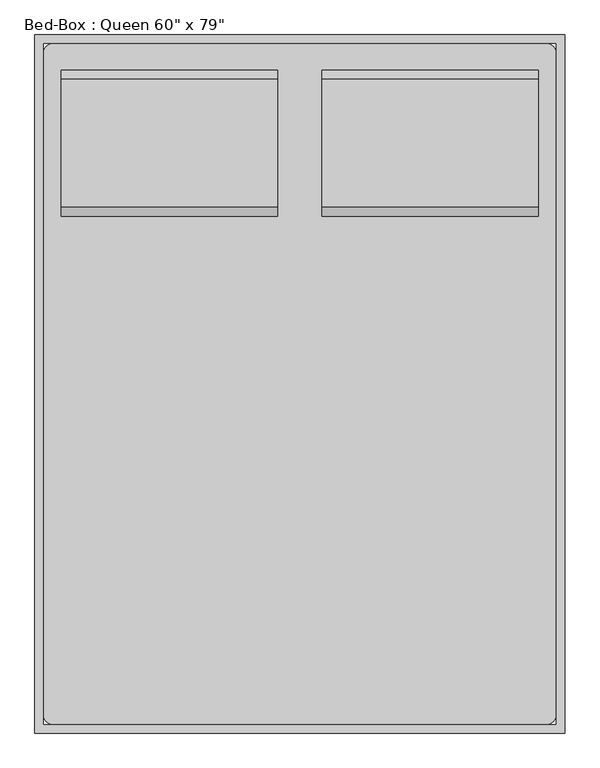
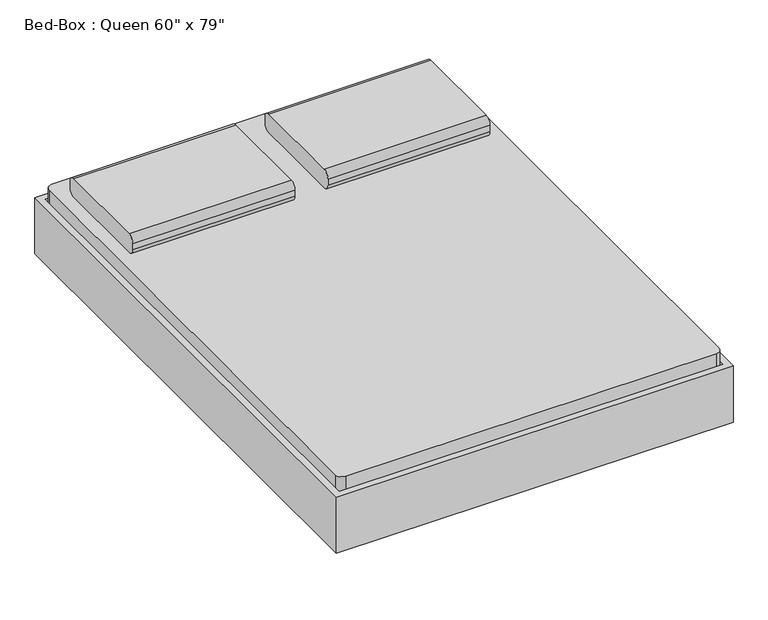
"""IFC4 building model written with IfcOpenShell, lengths in millimetres: furniture geometry."""

from ifc_helpers import new_model, si_unit, point, frame, frame_2d, origin, place, context, project, spatial, polyline, circle_curve, trimmed, segment, composite_curve, outline, extrude, source, transform, mapped, element, save
from ifc_brep_helpers import plane_surface, cylinder_surface, revolved_surface, advanced_brep


def furniture_0fd752b5(model_context):
    return source(origin(), model_context, "Body", "SolidModel", [
        extrude(outline(composite_curve([segment(polyline([(641.8704918, 406.4), (273.5704918, 406.4)]), True, "CONTINUOUS"), segment(trimmed(circle_curve(frame_2d((273.5704918, 431.8)), 25.4), [point((273.5704918, 406.4))], [point((248.1704918, 431.8))], False, "CARTESIAN"), True, "CONTINUOUS"), segment(polyline([(248.1704918, 431.8), (248.1704918, 457.2)]), True, "CONTINUOUS"), segment(trimmed(circle_curve(frame_2d((273.5704918, 457.2)), 25.4), [point((248.1704918, 457.2))], [point((273.5704918, 482.6))], False, "CARTESIAN"), True, "CONTINUOUS"), segment(polyline([(273.5704918, 482.6), (641.8704918, 482.6)]), True, "CONTINUOUS"), segment(trimmed(circle_curve(frame_2d((641.8704918, 457.2)), 25.4), [point((641.8704918, 482.6))], [point((667.2704918, 457.2))], False, "CARTESIAN"), True, "CONTINUOUS"), segment(polyline([(667.2704918, 457.2), (667.2704918, 431.8)]), True, "CONTINUOUS"), segment(trimmed(circle_curve(frame_2d((641.8704918, 431.8)), 25.4), [point((667.2704918, 431.8))], [point((641.8704918, 406.4))], False, "CARTESIAN"), True, "CONTINUOUS")], self_intersect=False)), frame((402.652459, 0.0, 0.0), z_axis=(1.0, 0.0, 0.0), x_axis=(0.0, 1.0, 0.0)), (0.0, 0.0, 1.0), 622.3),
        extrude(outline(composite_curve([segment(polyline([(641.8704918, 406.4), (273.5704918, 406.4)]), True, "CONTINUOUS"), segment(trimmed(circle_curve(frame_2d((273.5704918, 431.8)), 25.4), [point((273.5704918, 406.4))], [point((248.1704918, 431.8))], False, "CARTESIAN"), True, "CONTINUOUS"), segment(polyline([(248.1704918, 431.8), (248.1704918, 457.2)]), True, "CONTINUOUS"), segment(trimmed(circle_curve(frame_2d((273.5704918, 457.2)), 25.4), [point((248.1704918, 457.2))], [point((273.5704918, 482.6))], False, "CARTESIAN"), True, "CONTINUOUS"), segment(polyline([(273.5704918, 482.6), (641.8704918, 482.6)]), True, "CONTINUOUS"), segment(trimmed(circle_curve(frame_2d((641.8704918, 457.2)), 25.4), [point((641.8704918, 482.6))], [point((667.2704918, 457.2))], False, "CARTESIAN"), True, "CONTINUOUS"), segment(polyline([(667.2704918, 457.2), (667.2704918, 431.8)]), True, "CONTINUOUS"), segment(trimmed(circle_curve(frame_2d((641.8704918, 431.8)), 25.4), [point((667.2704918, 431.8))], [point((641.8704918, 406.4))], False, "CARTESIAN"), True, "CONTINUOUS")], self_intersect=False)), frame((-346.647541, 0.0, 0.0), z_axis=(1.0, 0.0, 0.0), x_axis=(0.0, 1.0, 0.0)), (0.0, 0.0, 1.0), 622.3),
        advanced_brep(
        [(-397.1231784, 514.8704918, 177.8), (-397.1231784, 438.6704918, 177.8), (-397.1231784, 438.6704918, 196.85), (-397.1231784, 514.8704918, 196.85), (-346.3231784, 514.8704918, 177.8), (-346.3231784, 438.6704918, 177.8), (-334.1869899, 438.6704918, 196.85), (-334.1869899, 514.8704918, 196.85), (-270.2523099, 514.8704918, 14.6654962), (-270.2523099, 438.6704918, 14.6654962), (-252.9871466, 438.6704918, 22.716374), (-252.9871466, 514.8704918, 22.716374), (-247.2320921, 438.6704918, 0.0), (-247.2320921, 514.8704918, 0.0), (-247.2320921, 438.6704918, 19.05), (-247.2320921, 514.8704918, 19.05), (-168.6195862, 514.8704918, 0.0), (-168.6195862, 438.6704918, 0.0), (-168.6195862, 438.6704918, 19.05), (-168.6195862, 514.8704918, 19.05), (-155.9195862, 438.6704918, 3.4029547), (-155.9195862, 514.8704918, 3.4029547), (-165.4445862, 438.6704918, 19.9007387), (-165.4445862, 514.8704918, 19.9007387), (-95.822541, 514.8704918, 38.1), (-95.822541, 438.6704918, 38.1), (-100.9269731, 438.6704918, 57.15), (-100.9269731, 514.8704918, 57.15), (774.4518216, 514.8704918, 38.1), (774.4518216, 438.6704918, 38.1), (779.5562537, 438.6704918, 57.15), (779.5562537, 514.8704918, 57.15), (834.5488669, 514.8704918, 3.4029547), (834.5488669, 438.6704918, 3.4029547), (844.0738669, 438.6704918, 19.9007387), (844.0738669, 514.8704918, 19.9007387), (847.2488669, 438.6704918, 0.0), (847.2488669, 514.8704918, 0.0), (847.2488669, 438.6704918, 19.05), (847.2488669, 514.8704918, 19.05), (925.8613728, 514.8704918, 0.0), (925.8613728, 438.6704918, 0.0), (925.8613728, 438.6704918, 19.05), (925.8613728, 514.8704918, 19.05), (948.8815906, 438.6704918, 14.6654962), (948.8815906, 514.8704918, 14.6654962), (931.6164272, 438.6704918, 22.716374), (931.6164272, 514.8704918, 22.716374), (1024.952459, 514.8704918, 177.8), (1024.952459, 438.6704918, 177.8), (1012.8162705, 438.6704918, 196.85), (1012.8162705, 514.8704918, 196.85), (1075.752459, 514.8704918, 177.8), (1075.752459, 514.8704918, 196.85), (1075.752459, 438.6704918, 196.85), (1075.752459, 438.6704918, 177.8)],
        [
            (0, 1),
            (1, 2),
            (2, 3),
            (3, 0),
            (0, 4),
            (4, 5),
            (5, 1),
            (5, 6),
            (6, 2),
            (6, 7),
            (7, 3),
            (7, 4),
            (4, 8),
            (8, 9),
            (9, 5),
            (9, 10),
            (10, 6),
            (10, 11),
            (11, 7),
            (11, 8),
            (12, 9, circle_curve(frame((-247.2320921, 438.6704918, 25.4), z_axis=(0.0, 1.0, 0.0), x_axis=(-0.9063077870366486, 0.0, -0.42261826174070233)), 25.4)),
            (8, 13, circle_curve(frame((-247.2320921, 514.8704918, 25.4), z_axis=(0.0, -1.0, 0.0), x_axis=(-0.9063077870366486, 0.0, -0.42261826174070233)), 25.4)),
            (13, 12),
            (14, 10, circle_curve(frame((-247.2320921, 438.6704918, 25.4), z_axis=(0.0, 1.0, 0.0), x_axis=(-0.9063077870366486, 0.0, -0.42261826174070233)), 6.35)),
            (12, 14),
            (15, 11, circle_curve(frame((-247.2320921, 514.8704918, 25.4), z_axis=(0.0, 1.0, 0.0), x_axis=(-0.9063077870366486, 0.0, -0.42261826174070233)), 6.35)),
            (14, 15),
            (15, 13),
            (13, 16),
            (16, 17),
            (17, 12),
            (17, 18),
            (18, 14),
            (18, 19),
            (19, 15),
            (19, 16),
            (20, 17, circle_curve(frame((-168.6195862, 438.6704918, 25.4), z_axis=(0.0, 1.0, 0.0), x_axis=(0.0, 0.0, -1.0)), 25.4)),
            (16, 21, circle_curve(frame((-168.6195862, 514.8704918, 25.4), z_axis=(0.0, -1.0, 0.0), x_axis=(0.0, 0.0, -1.0)), 25.4)),
            (21, 20),
            (22, 18, circle_curve(frame((-168.6195862, 438.6704918, 25.4), z_axis=(0.0, 1.0, 0.0), x_axis=(0.0, 0.0, -1.0)), 6.35)),
            (20, 22),
            (23, 19, circle_curve(frame((-168.6195862, 514.8704918, 25.4), z_axis=(0.0, 1.0, 0.0), x_axis=(0.0, 0.0, -1.0)), 6.35)),
            (22, 23),
            (23, 21),
            (21, 24),
            (24, 25),
            (25, 20),
            (25, 26),
            (26, 22),
            (26, 27),
            (27, 23),
            (27, 24),
            (24, 28),
            (28, 29),
            (29, 25),
            (29, 30),
            (30, 26),
            (30, 31),
            (31, 27),
            (31, 28),
            (28, 32),
            (32, 33),
            (33, 29),
            (33, 34),
            (34, 30),
            (34, 35),
            (35, 31),
            (35, 32),
            (36, 33, circle_curve(frame((847.2488669, 438.6704918, 25.4), z_axis=(0.0, 1.0, 0.0), x_axis=(-0.5000000000000463, 0.0, -0.8660254037844118)), 25.4)),
            (32, 37, circle_curve(frame((847.2488669, 514.8704918, 25.4), z_axis=(0.0, -1.0, 0.0), x_axis=(-0.5000000000000463, 0.0, -0.8660254037844118)), 25.4)),
            (37, 36),
            (38, 34, circle_curve(frame((847.2488669, 438.6704918, 25.4), z_axis=(0.0, 1.0, 0.0), x_axis=(-0.5000000000000463, 0.0, -0.8660254037844118)), 6.35)),
            (36, 38),
            (39, 35, circle_curve(frame((847.2488669, 514.8704918, 25.4), z_axis=(0.0, 1.0, 0.0), x_axis=(-0.5000000000000463, 0.0, -0.8660254037844118)), 6.35)),
            (38, 39),
            (39, 37),
            (37, 40),
            (40, 41),
            (41, 36),
            (41, 42),
            (42, 38),
            (42, 43),
            (43, 39),
            (43, 40),
            (44, 41, circle_curve(frame((925.8613728, 438.6704918, 25.4), z_axis=(0.0, 1.0, 0.0), x_axis=(0.0, 0.0, -1.0)), 25.4)),
            (40, 45, circle_curve(frame((925.8613728, 514.8704918, 25.4), z_axis=(0.0, -1.0, 0.0), x_axis=(0.0, 0.0, -1.0)), 25.4)),
            (45, 44),
            (46, 42, circle_curve(frame((925.8613728, 438.6704918, 25.4), z_axis=(0.0, 1.0, 0.0), x_axis=(0.0, 0.0, -1.0)), 6.35)),
            (44, 46),
            (47, 43, circle_curve(frame((925.8613728, 514.8704918, 25.4), z_axis=(0.0, 1.0, 0.0), x_axis=(0.0, 0.0, -1.0)), 6.35)),
            (46, 47),
            (47, 45),
            (45, 48),
            (48, 49),
            (49, 44),
            (49, 50),
            (50, 46),
            (50, 51),
            (51, 47),
            (51, 48),
            (52, 53),
            (53, 54),
            (54, 55),
            (55, 52),
            (48, 52),
            (55, 49),
            (54, 50),
            (53, 51),
        ],
        [
            plane_surface(frame((-397.1231784, 768.8704918, -152.9490627), z_axis=(-1.0, 0.0, 0.0), x_axis=(0.0, 1.0, 0.0))),
            plane_surface(frame((-397.1231784, 514.8704918, 177.8), z_axis=(0.0, 0.0, -1.0), x_axis=(1.0, 0.0, 0.0))),
            plane_surface(frame((-397.1231784, 438.6704918, 177.8), z_axis=(0.0, -1.0, 0.0), x_axis=(1.0, 0.0, 0.0))),
            plane_surface(frame((-397.1231784, 438.6704918, 196.85), z_axis=(0.0, 0.0, 1.0), x_axis=(1.0, 0.0, 0.0))),
            plane_surface(frame((-397.1231784, 514.8704918, 196.85), z_axis=(0.0, 1.0, 0.0), x_axis=(1.0, 0.0, 0.0))),
            plane_surface(frame((-346.3231784, 514.8704918, 177.8), z_axis=(-0.9063077870366485, 0.0, -0.4226182617407027), x_axis=(0.4226182617407027, 0.0, -0.9063077870366485))),
            plane_surface(frame((-346.3231784, 438.6704918, 177.8), z_axis=(0.0, -1.0, 0.0), x_axis=(0.4226182617407025, 0.0, -0.9063077870366486))),
            plane_surface(frame((-334.1869899, 438.6704918, 196.85), z_axis=(0.9063077870366484, 0.0, 0.4226182617407028), x_axis=(0.4226182617407028, 0.0, -0.9063077870366484))),
            plane_surface(frame((-334.1869899, 514.8704918, 196.85), z_axis=(0.0, 1.0, 0.0), x_axis=(0.42261826174070277, 0.0, -0.9063077870366485))),
            cylinder_surface(frame((-247.2320921, 768.8704918, 25.4), z_axis=(0.0, -1.0, 0.0), x_axis=(-0.9063077870366486, 0.0, -0.42261826174070233)), 25.4),
            plane_surface(frame((-247.2320921, 438.6704918, 25.4), z_axis=(0.0, -1.0, 0.0), x_axis=(-0.9063077870366486, 0.0, -0.42261826174070233))),
            revolved_surface(polyline([(-252.9871465476827, 438.6704918, 22.71637403794654), (-252.9871465476827, 514.8704918, 22.71637403794654)]), (-247.2320921, 768.8704918, 25.4), (0.0, -1.0, 0.0)),
            plane_surface(frame((-247.2320921, 514.8704918, 25.4), z_axis=(0.0, 1.0, 0.0), x_axis=(-0.9063077870366486, 0.0, -0.42261826174070233))),
            plane_surface(frame((-247.2320921, 514.8704918, 0.0), z_axis=(0.0, 0.0, -1.0), x_axis=(1.0, 0.0, 0.0))),
            plane_surface(frame((-247.2320921, 438.6704918, 0.0), z_axis=(0.0, -1.0, 0.0), x_axis=(1.0, 0.0, 0.0))),
            plane_surface(frame((-247.2320921, 438.6704918, 19.05), z_axis=(0.0, 0.0, 1.0), x_axis=(1.0, 0.0, 0.0))),
            plane_surface(frame((-247.2320921, 514.8704918, 19.05), z_axis=(0.0, 1.0, 0.0), x_axis=(1.0, 0.0, 0.0))),
            cylinder_surface(frame((-168.6195862, 768.8704918, 25.4), z_axis=(0.0, -1.0, 0.0), x_axis=(0.0, 0.0, -1.0)), 25.4),
            plane_surface(frame((-168.6195862, 438.6704918, 25.4), z_axis=(0.0, -1.0, 0.0), x_axis=(0.0, 0.0, -1.0))),
            revolved_surface(polyline([(-168.6195862, 438.6704918, 19.049999999999997), (-168.6195862, 514.8704918, 19.049999999999997)]), (-168.6195862, 768.8704918, 25.4), (0.0, -1.0, 0.0)),
            plane_surface(frame((-168.6195862, 514.8704918, 25.4), z_axis=(0.0, 1.0, 0.0), x_axis=(0.0, 0.0, -1.0))),
            plane_surface(frame((-155.9195862, 514.8704918, 3.4029547), z_axis=(0.49999999999988004, 0.0, -0.866025403784508), x_axis=(0.866025403784508, 0.0, 0.49999999999988004))),
            plane_surface(frame((-155.9195862, 438.6704918, 3.4029547), z_axis=(0.0, -1.0, 0.0), x_axis=(0.8660254037845078, 0.0, 0.49999999999988026))),
            plane_surface(frame((-165.4445862, 438.6704918, 19.9007387), z_axis=(-0.4999999999998799, 0.0, 0.866025403784508), x_axis=(0.866025403784508, 0.0, 0.4999999999998799))),
            plane_surface(frame((-165.4445862, 514.8704918, 19.9007387), z_axis=(0.0, 1.0, 0.0), x_axis=(0.8660254037845075, 0.0, 0.49999999999988076))),
            plane_surface(frame((-95.822541, 514.8704918, 38.1), z_axis=(0.0, 0.0, -1.0), x_axis=(1.0, 0.0, 0.0))),
            plane_surface(frame((-95.822541, 438.6704918, 38.1), z_axis=(0.0, -1.0, 0.0), x_axis=(1.0, 0.0, 0.0))),
            plane_surface(frame((-100.9269731, 438.6704918, 57.15), z_axis=(0.0, 0.0, 1.0), x_axis=(1.0, 0.0, 0.0))),
            plane_surface(frame((-100.9269731, 514.8704918, 57.15), z_axis=(0.0, 1.0, 0.0), x_axis=(1.0, 0.0, 0.0))),
            plane_surface(frame((774.4518216, 514.8704918, 38.1), z_axis=(-0.5000000000000455, 0.0, -0.8660254037844125), x_axis=(0.8660254037844125, 0.0, -0.5000000000000455))),
            plane_surface(frame((774.4518216, 438.6704918, 38.1), z_axis=(0.0, -1.0, 0.0), x_axis=(0.866025403784412, 0.0, -0.5000000000000463))),
            plane_surface(frame((779.5562537, 438.6704918, 57.15), z_axis=(0.5000000000000466, 0.0, 0.8660254037844117), x_axis=(0.8660254037844117, 0.0, -0.5000000000000466))),
            plane_surface(frame((779.5562537, 514.8704918, 57.15), z_axis=(0.0, 1.0, 0.0), x_axis=(0.8660254037844115, 0.0, -0.5000000000000471))),
            cylinder_surface(frame((847.2488669, 768.8704918, 25.4), z_axis=(0.0, -1.0, 0.0), x_axis=(-0.5000000000000463, 0.0, -0.8660254037844118)), 25.4),
            plane_surface(frame((847.2488669, 438.6704918, 25.4), z_axis=(0.0, -1.0000000000000002, 0.0), x_axis=(-0.5000000000000464, 0.0, -0.866025403784412))),
            revolved_surface(polyline([(844.0738668999998, 438.6704918, 19.90073868596898), (844.0738668999998, 514.8704918, 19.90073868596898)]), (847.2488669, 768.8704918, 25.4), (0.0, -1.0, 0.0)),
            plane_surface(frame((847.2488669, 514.8704918, 25.4), z_axis=(0.0, 1.0000000000000002, 0.0), x_axis=(-0.5000000000000464, 0.0, -0.866025403784412))),
            plane_surface(frame((847.2488669, 514.8704918, 0.0), z_axis=(0.0, 0.0, -1.0), x_axis=(1.0, 0.0, 0.0))),
            plane_surface(frame((847.2488669, 438.6704918, 0.0), z_axis=(0.0, -1.0, 0.0), x_axis=(1.0, 0.0, 0.0))),
            plane_surface(frame((847.2488669, 438.6704918, 19.05), z_axis=(0.0, 0.0, 1.0), x_axis=(1.0, 0.0, 0.0))),
            plane_surface(frame((847.2488669, 514.8704918, 19.05), z_axis=(0.0, 1.0, 0.0), x_axis=(1.0, 0.0, 0.0))),
            cylinder_surface(frame((925.8613728, 768.8704918, 25.4), z_axis=(0.0, -1.0, 0.0), x_axis=(0.0, 0.0, -1.0)), 25.4),
            plane_surface(frame((925.8613728, 438.6704918, 25.4), z_axis=(0.0, -1.0, 0.0), x_axis=(0.0, 0.0, -1.0))),
            revolved_surface(polyline([(925.8613728, 438.6704918, 19.049999999999997), (925.8613728, 514.8704918, 19.049999999999997)]), (925.8613728, 768.8704918, 25.4), (0.0, -1.0, 0.0)),
            plane_surface(frame((925.8613728, 514.8704918, 25.4), z_axis=(0.0, 1.0, 0.0), x_axis=(0.0, 0.0, -1.0))),
            plane_surface(frame((948.8815906, 514.8704918, 14.6654962), z_axis=(0.90630778703668, 0.0, -0.42261826174063527), x_axis=(0.42261826174063527, 0.0, 0.90630778703668))),
            plane_surface(frame((948.8815906, 438.6704918, 14.6654962), z_axis=(0.0, -1.0, 0.0), x_axis=(0.42261826174063566, 0.0, 0.9063077870366797))),
            plane_surface(frame((931.6164272, 438.6704918, 22.716374), z_axis=(-0.9063077870366801, 0.0, 0.4226182617406349), x_axis=(0.4226182617406349, 0.0, 0.9063077870366801))),
            plane_surface(frame((931.6164272, 514.8704918, 22.716374), z_axis=(0.0, 1.0, 0.0), x_axis=(0.4226182617406353, 0.0, 0.9063077870366799))),
            plane_surface(frame((1075.752459, 768.8704918, -152.9490627), z_axis=(1.0, 0.0, 0.0), x_axis=(0.0, 1.0, 0.0))),
            plane_surface(frame((1024.952459, 514.8704918, 177.8), z_axis=(0.0, 0.0, -1.0), x_axis=(1.0, 0.0, 0.0))),
            plane_surface(frame((1024.952459, 438.6704918, 177.8), z_axis=(0.0, -1.0, 0.0), x_axis=(1.0, 0.0, 0.0))),
            plane_surface(frame((1012.8162705, 438.6704918, 196.85), z_axis=(0.0, 0.0, 1.0), x_axis=(1.0, 0.0, 0.0))),
            plane_surface(frame((1012.8162705, 514.8704918, 196.85), z_axis=(0.0, 1.0, 0.0), x_axis=(1.0, 0.0, 0.0))),
        ],
        [
            (0, [[1, 2, 3, 4]]),
            (1, [[-1, 5, 6, 7]]),
            (2, [[-2, -7, 8, 9]]),
            (3, [[-3, -9, 10, 11]]),
            (4, [[-4, -11, 12, -5]]),
            (5, [[-6, 13, 14, 15]]),
            (6, [[-8, -15, 16, 17]]),
            (7, [[-10, -17, 18, 19]]),
            (8, [[-12, -19, 20, -13]]),
            (9, [[21, -14, 22, 23]]),
            (10, [[24, -16, -21, 25]]),
            (11, [[26, -18, -24, 27]]),
            (12, [[-22, -20, -26, 28]]),
            (13, [[-23, 29, 30, 31]]),
            (14, [[-25, -31, 32, 33]]),
            (15, [[-27, -33, 34, 35]]),
            (16, [[-28, -35, 36, -29]]),
            (17, [[37, -30, 38, 39]]),
            (18, [[40, -32, -37, 41]]),
            (19, [[42, -34, -40, 43]]),
            (20, [[-38, -36, -42, 44]]),
            (21, [[-39, 45, 46, 47]]),
            (22, [[-41, -47, 48, 49]]),
            (23, [[-43, -49, 50, 51]]),
            (24, [[-44, -51, 52, -45]]),
            (25, [[-46, 53, 54, 55]]),
            (26, [[-48, -55, 56, 57]]),
            (27, [[-50, -57, 58, 59]]),
            (28, [[-52, -59, 60, -53]]),
            (29, [[-54, 61, 62, 63]]),
            (30, [[-56, -63, 64, 65]]),
            (31, [[-58, -65, 66, 67]]),
            (32, [[-60, -67, 68, -61]]),
            (33, [[69, -62, 70, 71]]),
            (34, [[72, -64, -69, 73]]),
            (35, [[74, -66, -72, 75]]),
            (36, [[-70, -68, -74, 76]]),
            (37, [[-71, 77, 78, 79]]),
            (38, [[-73, -79, 80, 81]]),
            (39, [[-75, -81, 82, 83]]),
            (40, [[-76, -83, 84, -77]]),
            (41, [[85, -78, 86, 87]]),
            (42, [[88, -80, -85, 89]]),
            (43, [[90, -82, -88, 91]]),
            (44, [[-86, -84, -90, 92]]),
            (45, [[-87, 93, 94, 95]]),
            (46, [[-89, -95, 96, 97]]),
            (47, [[-91, -97, 98, 99]]),
            (48, [[-92, -99, 100, -93]]),
            (49, [[101, 102, 103, 104]]),
            (50, [[-94, 105, -104, 106]]),
            (51, [[-96, -106, -103, 107]]),
            (52, [[-98, -107, -102, 108]]),
            (53, [[-100, -108, -101, -105]]),
        ],
    ),
        extrude(outline(composite_curve([segment(polyline([(-372.047541, 743.4704918), (1050.352459, 743.4704918)]), True, "CONTINUOUS"), segment(trimmed(circle_curve(frame_2d((1050.352459, 718.0704918)), 25.4), [point((1050.352459, 743.4704918))], [point((1075.752459, 718.0704918))], False, "CARTESIAN"), True, "CONTINUOUS"), segment(polyline([(1075.752459, 718.0704918), (1075.752459, -1186.9295082)]), True, "CONTINUOUS"), segment(trimmed(circle_curve(frame_2d((1050.352459, -1186.9295082)), 25.4), [point((1075.752459, -1186.9295082))], [point((1050.352459, -1212.3295082))], False, "CARTESIAN"), True, "CONTINUOUS"), segment(polyline([(1050.352459, -1212.3295082), (-372.047541, -1212.3295082)]), True, "CONTINUOUS"), segment(trimmed(circle_curve(frame_2d((-372.047541, -1186.9295082)), 25.4), [point((-372.047541, -1212.3295082))], [point((-397.447541, -1186.9295082))], False, "CARTESIAN"), True, "CONTINUOUS"), segment(polyline([(-397.447541, -1186.9295082), (-397.447541, 718.0704918)]), True, "CONTINUOUS"), segment(trimmed(circle_curve(frame_2d((-372.047541, 718.0704918)), 25.4), [point((-397.447541, 718.0704918))], [point((-372.047541, 743.4704918))], False, "CARTESIAN"), True, "CONTINUOUS")], self_intersect=False)), frame((0.0, 0.0, 203.2), z_axis=(0.0, 0.0, 1.0), x_axis=(1.0, 0.0, 0.0)), (0.0, 0.0, 1.0), 203.2),
        advanced_brep(
        [(-397.447541, -932.9295082, 196.85), (-397.447541, -932.9295082, 177.8), (-397.447541, -1009.1295082, 177.8), (-397.447541, -1009.1295082, 196.85), (-334.5113525, -932.9295082, 196.85), (-346.647541, -932.9295082, 177.8), (-346.647541, -1009.1295082, 177.8), (-334.5113525, -1009.1295082, 196.85), (-253.3115092, -932.9295082, 22.716374), (-270.5766725, -932.9295082, 14.6654962), (-270.5766725, -1009.1295082, 14.6654962), (-253.3115092, -1009.1295082, 22.716374), (-247.5564547, -932.9295082, 0.0), (-247.5564547, -932.9295082, 19.05), (-247.5564547, -1009.1295082, 0.0), (-247.5564547, -1009.1295082, 19.05), (-168.9439489, -932.9295082, 19.05), (-168.9439489, -932.9295082, 0.0), (-168.9439489, -1009.1295082, 0.0), (-168.9439489, -1009.1295082, 19.05), (-156.2439489, -932.9295082, 3.4029547), (-165.7689489, -932.9295082, 19.9007387), (-156.2439489, -1009.1295082, 3.4029547), (-165.7689489, -1009.1295082, 19.9007387), (-101.2513357, -932.9295082, 57.15), (-96.1469036, -932.9295082, 38.1), (-96.1469036, -1009.1295082, 38.1), (-101.2513357, -1009.1295082, 57.15), (779.5562537, -932.9295082, 57.15), (774.4518216, -932.9295082, 38.1), (774.4518216, -1009.1295082, 38.1), (779.5562537, -1009.1295082, 57.15), (844.0738669, -932.9295082, 19.9007387), (834.5488669, -932.9295082, 3.4029547), (834.5488669, -1009.1295082, 3.4029547), (844.0738669, -1009.1295082, 19.9007387), (847.2488669, -932.9295082, 0.0), (847.2488669, -932.9295082, 19.05), (847.2488669, -1009.1295082, 0.0), (847.2488669, -1009.1295082, 19.05), (925.8613728, -932.9295082, 19.05), (925.8613728, -932.9295082, 0.0), (925.8613728, -1009.1295082, 0.0), (925.8613728, -1009.1295082, 19.05), (948.8815906, -932.9295082, 14.6654962), (931.6164272, -932.9295082, 22.716374), (948.8815906, -1009.1295082, 14.6654962), (931.6164272, -1009.1295082, 22.716374), (1012.8162705, -932.9295082, 196.85), (1024.952459, -932.9295082, 177.8), (1024.952459, -1009.1295082, 177.8), (1012.8162705, -1009.1295082, 196.85), (1075.752459, -932.9295082, 196.85), (1075.752459, -1009.1295082, 196.85), (1075.752459, -1009.1295082, 177.8), (1075.752459, -932.9295082, 177.8)],
        [
            (0, 1),
            (1, 2),
            (2, 3),
            (3, 0),
            (0, 4),
            (4, 5),
            (5, 1),
            (5, 6),
            (6, 2),
            (6, 7),
            (7, 3),
            (7, 4),
            (4, 8),
            (8, 9),
            (9, 5),
            (9, 10),
            (10, 6),
            (10, 11),
            (11, 7),
            (11, 8),
            (12, 9, circle_curve(frame((-247.5564547, -932.9295082, 25.4), z_axis=(0.0, 1.0, 0.0), x_axis=(-0.906307787036663, 0.0, -0.4226182617406713)), 25.4)),
            (8, 13, circle_curve(frame((-247.5564547, -932.9295082, 25.4), z_axis=(0.0, -1.0, 0.0), x_axis=(-0.906307787036663, 0.0, -0.4226182617406713)), 6.35)),
            (13, 12),
            (14, 10, circle_curve(frame((-247.5564547, -1009.1295082, 25.4), z_axis=(0.0, 1.0, 0.0), x_axis=(-0.906307787036663, 0.0, -0.4226182617406713)), 25.4)),
            (12, 14),
            (15, 11, circle_curve(frame((-247.5564547, -1009.1295082, 25.4), z_axis=(0.0, 1.0, 0.0), x_axis=(-0.906307787036663, 0.0, -0.4226182617406713)), 6.35)),
            (14, 15),
            (15, 13),
            (13, 16),
            (16, 17),
            (17, 12),
            (17, 18),
            (18, 14),
            (18, 19),
            (19, 15),
            (19, 16),
            (20, 17, circle_curve(frame((-168.9439489, -932.9295082, 25.4), z_axis=(0.0, 1.0, 0.0), x_axis=(0.0, 0.0, -1.0)), 25.4)),
            (16, 21, circle_curve(frame((-168.9439489, -932.9295082, 25.4), z_axis=(0.0, -1.0, 0.0), x_axis=(0.0, 0.0, -1.0)), 6.35)),
            (21, 20),
            (22, 18, circle_curve(frame((-168.9439489, -1009.1295082, 25.4), z_axis=(0.0, 1.0, 0.0), x_axis=(0.0, 0.0, -1.0)), 25.4)),
            (20, 22),
            (23, 19, circle_curve(frame((-168.9439489, -1009.1295082, 25.4), z_axis=(0.0, 1.0, 0.0), x_axis=(0.0, 0.0, -1.0)), 6.35)),
            (22, 23),
            (23, 21),
            (21, 24),
            (24, 25),
            (25, 20),
            (25, 26),
            (26, 22),
            (26, 27),
            (27, 23),
            (27, 24),
            (24, 28),
            (28, 29),
            (29, 25),
            (29, 30),
            (30, 26),
            (30, 31),
            (31, 27),
            (31, 28),
            (28, 32),
            (32, 33),
            (33, 29),
            (33, 34),
            (34, 30),
            (34, 35),
            (35, 31),
            (35, 32),
            (36, 33, circle_curve(frame((847.2488669, -932.9295082, 25.4), z_axis=(0.0, 1.0, 0.0), x_axis=(-0.5000000000000479, 0.0, -0.866025403784411)), 25.4)),
            (32, 37, circle_curve(frame((847.2488669, -932.9295082, 25.4), z_axis=(0.0, -1.0, 0.0), x_axis=(-0.5000000000000479, 0.0, -0.866025403784411)), 6.35)),
            (37, 36),
            (38, 34, circle_curve(frame((847.2488669, -1009.1295082, 25.4), z_axis=(0.0, 1.0, 0.0), x_axis=(-0.5000000000000479, 0.0, -0.866025403784411)), 25.4)),
            (36, 38),
            (39, 35, circle_curve(frame((847.2488669, -1009.1295082, 25.4), z_axis=(0.0, 1.0, 0.0), x_axis=(-0.5000000000000479, 0.0, -0.866025403784411)), 6.35)),
            (38, 39),
            (39, 37),
            (37, 40),
            (40, 41),
            (41, 36),
            (41, 42),
            (42, 38),
            (42, 43),
            (43, 39),
            (43, 40),
            (44, 41, circle_curve(frame((925.8613728, -932.9295082, 25.4), z_axis=(0.0, 1.0, 0.0), x_axis=(0.0, 0.0, -1.0)), 25.4)),
            (40, 45, circle_curve(frame((925.8613728, -932.9295082, 25.4), z_axis=(0.0, -1.0, 0.0), x_axis=(0.0, 0.0, -1.0)), 6.35)),
            (45, 44),
            (46, 42, circle_curve(frame((925.8613728, -1009.1295082, 25.4), z_axis=(0.0, 1.0, 0.0), x_axis=(0.0, 0.0, -1.0)), 25.4)),
            (44, 46),
            (47, 43, circle_curve(frame((925.8613728, -1009.1295082, 25.4), z_axis=(0.0, 1.0, 0.0), x_axis=(0.0, 0.0, -1.0)), 6.35)),
            (46, 47),
            (47, 45),
            (45, 48),
            (48, 49),
            (49, 44),
            (49, 50),
            (50, 46),
            (50, 51),
            (51, 47),
            (51, 48),
            (52, 53),
            (53, 54),
            (54, 55),
            (55, 52),
            (48, 52),
            (55, 49),
            (54, 50),
            (53, 51),
        ],
        [
            plane_surface(frame((-397.447541, -1237.7295082, -127.5947323), z_axis=(-1.0, 0.0, 0.0), x_axis=(0.0, 1.0, 0.0))),
            plane_surface(frame((-397.447541, -932.9295082, 196.85), z_axis=(0.0, 1.0, 0.0), x_axis=(1.0, 0.0, 0.0))),
            plane_surface(frame((-397.447541, -932.9295082, 177.8), z_axis=(0.0, 0.0, -1.0), x_axis=(1.0, 0.0, 0.0))),
            plane_surface(frame((-397.447541, -1009.1295082, 177.8), z_axis=(0.0, -1.0, 0.0), x_axis=(1.0, 0.0, 0.0))),
            plane_surface(frame((-397.447541, -1009.1295082, 196.85), z_axis=(0.0, 0.0, 1.0), x_axis=(1.0, 0.0, 0.0))),
            plane_surface(frame((-334.5113525, -932.9295082, 196.85), z_axis=(0.0, 1.0, 0.0), x_axis=(0.4226182617406707, 0.0, -0.9063077870366634))),
            plane_surface(frame((-346.647541, -932.9295082, 177.8), z_axis=(-0.9063077870366635, 0.0, -0.4226182617406707), x_axis=(0.4226182617406707, 0.0, -0.9063077870366635))),
            plane_surface(frame((-346.647541, -1009.1295082, 177.8), z_axis=(0.0, -1.0, 0.0), x_axis=(0.422618261740671, 0.0, -0.9063077870366633))),
            plane_surface(frame((-334.5113525, -1009.1295082, 196.85), z_axis=(0.9063077870366633, 0.0, 0.42261826174067113), x_axis=(0.42261826174067113, 0.0, -0.9063077870366633))),
            plane_surface(frame((-247.5564547, -932.9295082, 25.4), z_axis=(0.0, 1.0, 0.0), x_axis=(-0.906307787036663, 0.0, -0.4226182617406713))),
            cylinder_surface(frame((-247.5564547, -1237.7295082, 25.4), z_axis=(0.0, -1.0, 0.0), x_axis=(-0.906307787036663, 0.0, -0.4226182617406713)), 25.4),
            plane_surface(frame((-247.5564547, -1009.1295082, 25.4), z_axis=(0.0, -1.0, 0.0), x_axis=(-0.906307787036663, 0.0, -0.4226182617406713))),
            revolved_surface(polyline([(-253.3115091476828, -1009.1295082, 22.716374037946736), (-253.3115091476828, -932.9295082, 22.716374037946736)]), (-247.5564547, -1237.7295082, 25.4), (0.0, -1.0, 0.0)),
            plane_surface(frame((-247.5564547, -932.9295082, 19.05), z_axis=(0.0, 1.0, 0.0), x_axis=(1.0, 0.0, 0.0))),
            plane_surface(frame((-247.5564547, -932.9295082, 0.0), z_axis=(0.0, 0.0, -1.0), x_axis=(1.0, 0.0, 0.0))),
            plane_surface(frame((-247.5564547, -1009.1295082, 0.0), z_axis=(0.0, -1.0, 0.0), x_axis=(1.0, 0.0, 0.0))),
            plane_surface(frame((-247.5564547, -1009.1295082, 19.05), z_axis=(0.0, 0.0, 1.0), x_axis=(1.0, 0.0, 0.0))),
            plane_surface(frame((-168.9439489, -932.9295082, 25.4), z_axis=(0.0, 1.0, 0.0), x_axis=(0.0, 0.0, -1.0))),
            cylinder_surface(frame((-168.9439489, -1237.7295082, 25.4), z_axis=(0.0, -1.0, 0.0), x_axis=(0.0, 0.0, -1.0)), 25.4),
            plane_surface(frame((-168.9439489, -1009.1295082, 25.4), z_axis=(0.0, -1.0, 0.0), x_axis=(0.0, 0.0, -1.0))),
            revolved_surface(polyline([(-168.9439489, -1009.1295082, 19.049999999999997), (-168.9439489, -932.9295082, 19.049999999999997)]), (-168.9439489, -1237.7295082, 25.4), (0.0, -1.0, 0.0)),
            plane_surface(frame((-165.7689489, -932.9295082, 19.9007387), z_axis=(0.0, 1.0, 0.0), x_axis=(0.8660254037844788, 0.0, 0.4999999999999306))),
            plane_surface(frame((-156.2439489, -932.9295082, 3.4029547), z_axis=(0.49999999999993017, 0.0, -0.866025403784479), x_axis=(0.866025403784479, 0.0, 0.49999999999993017))),
            plane_surface(frame((-156.2439489, -1009.1295082, 3.4029547), z_axis=(0.0, -1.0, 0.0), x_axis=(0.8660254037844785, 0.0, 0.49999999999993106))),
            plane_surface(frame((-165.7689489, -1009.1295082, 19.9007387), z_axis=(-0.4999999999999309, 0.0, 0.8660254037844786), x_axis=(0.8660254037844786, 0.0, 0.4999999999999309))),
            plane_surface(frame((-101.2513357, -932.9295082, 57.15), z_axis=(0.0, 1.0, 0.0), x_axis=(1.0, 0.0, 0.0))),
            plane_surface(frame((-96.1469036, -932.9295082, 38.1), z_axis=(0.0, 0.0, -1.0), x_axis=(1.0, 0.0, 0.0))),
            plane_surface(frame((-96.1469036, -1009.1295082, 38.1), z_axis=(0.0, -1.0, 0.0), x_axis=(1.0, 0.0, 0.0))),
            plane_surface(frame((-101.2513357, -1009.1295082, 57.15), z_axis=(0.0, 0.0, 1.0), x_axis=(1.0, 0.0, 0.0))),
            plane_surface(frame((779.5562537, -932.9295082, 57.15), z_axis=(0.0, 1.0000000000000002, 0.0), x_axis=(0.8660254037844106, 0.0, -0.5000000000000487))),
            plane_surface(frame((774.4518216, -932.9295082, 38.1), z_axis=(-0.5000000000000477, 0.0, -0.8660254037844112), x_axis=(0.8660254037844112, 0.0, -0.5000000000000477))),
            plane_surface(frame((774.4518216, -1009.1295082, 38.1), z_axis=(0.0, -1.0000000000000002, 0.0), x_axis=(0.8660254037844105, 0.0, -0.500000000000049))),
            plane_surface(frame((779.5562537, -1009.1295082, 57.15), z_axis=(0.5000000000000498, 0.0, 0.8660254037844098), x_axis=(0.8660254037844098, 0.0, -0.5000000000000498))),
            plane_surface(frame((847.2488669, -932.9295082, 25.4), z_axis=(0.0, 1.0000000000000002, 0.0), x_axis=(-0.500000000000048, 0.0, -0.8660254037844111))),
            cylinder_surface(frame((847.2488669, -1237.7295082, 25.4), z_axis=(0.0, -1.0, 0.0), x_axis=(-0.5000000000000479, 0.0, -0.866025403784411)), 25.4),
            plane_surface(frame((847.2488669, -1009.1295082, 25.4), z_axis=(0.0, -1.0000000000000002, 0.0), x_axis=(-0.500000000000048, 0.0, -0.8660254037844111))),
            revolved_surface(polyline([(844.0738668999998, -1009.1295082, 19.90073868596899), (844.0738668999998, -932.9295082, 19.90073868596899)]), (847.2488669, -1237.7295082, 25.4), (0.0, -1.0, 0.0)),
            plane_surface(frame((847.2488669, -932.9295082, 19.05), z_axis=(0.0, 1.0, 0.0), x_axis=(1.0, 0.0, 0.0))),
            plane_surface(frame((847.2488669, -932.9295082, 0.0), z_axis=(0.0, 0.0, -1.0), x_axis=(1.0, 0.0, 0.0))),
            plane_surface(frame((847.2488669, -1009.1295082, 0.0), z_axis=(0.0, -1.0, 0.0), x_axis=(1.0, 0.0, 0.0))),
            plane_surface(frame((847.2488669, -1009.1295082, 19.05), z_axis=(0.0, 0.0, 1.0), x_axis=(1.0, 0.0, 0.0))),
            plane_surface(frame((925.8613728, -932.9295082, 25.4), z_axis=(0.0, 1.0, 0.0), x_axis=(0.0, 0.0, -1.0))),
            cylinder_surface(frame((925.8613728, -1237.7295082, 25.4), z_axis=(0.0, -1.0, 0.0), x_axis=(0.0, 0.0, -1.0)), 25.4),
            plane_surface(frame((925.8613728, -1009.1295082, 25.4), z_axis=(0.0, -1.0, 0.0), x_axis=(0.0, 0.0, -1.0))),
            revolved_surface(polyline([(925.8613728, -1009.1295082, 19.049999999999997), (925.8613728, -932.9295082, 19.049999999999997)]), (925.8613728, -1237.7295082, 25.4), (0.0, -1.0, 0.0)),
            plane_surface(frame((931.6164272, -932.9295082, 22.716374), z_axis=(0.0, 1.0, 0.0), x_axis=(0.4226182617405411, 0.0, 0.9063077870367238))),
            plane_surface(frame((948.8815906, -932.9295082, 14.6654962), z_axis=(0.9063077870367237, 0.0, -0.4226182617405414), x_axis=(0.4226182617405414, 0.0, 0.9063077870367237))),
            plane_surface(frame((948.8815906, -1009.1295082, 14.6654962), z_axis=(0.0, -1.0, 0.0), x_axis=(0.42261826174054123, 0.0, 0.9063077870367238))),
            plane_surface(frame((931.6164272, -1009.1295082, 22.716374), z_axis=(-0.9063077870367237, 0.0, 0.4226182617405414), x_axis=(0.4226182617405414, 0.0, 0.9063077870367237))),
            plane_surface(frame((1075.752459, -1237.7295082, -127.5947323), z_axis=(1.0, 0.0, 0.0), x_axis=(0.0, 1.0, 0.0))),
            plane_surface(frame((1012.8162705, -932.9295082, 196.85), z_axis=(0.0, 1.0, 0.0), x_axis=(1.0, 0.0, 0.0))),
            plane_surface(frame((1024.952459, -932.9295082, 177.8), z_axis=(0.0, 0.0, -1.0), x_axis=(1.0, 0.0, 0.0))),
            plane_surface(frame((1024.952459, -1009.1295082, 177.8), z_axis=(0.0, -1.0, 0.0), x_axis=(1.0, 0.0, 0.0))),
            plane_surface(frame((1012.8162705, -1009.1295082, 196.85), z_axis=(0.0, 0.0, 1.0), x_axis=(1.0, 0.0, 0.0))),
        ],
        [
            (0, [[1, 2, 3, 4]]),
            (1, [[-1, 5, 6, 7]]),
            (2, [[-2, -7, 8, 9]]),
            (3, [[-3, -9, 10, 11]]),
            (4, [[-4, -11, 12, -5]]),
            (5, [[-6, 13, 14, 15]]),
            (6, [[-8, -15, 16, 17]]),
            (7, [[-10, -17, 18, 19]]),
            (8, [[-12, -19, 20, -13]]),
            (9, [[21, -14, 22, 23]]),
            (10, [[24, -16, -21, 25]]),
            (11, [[26, -18, -24, 27]]),
            (12, [[-22, -20, -26, 28]]),
            (13, [[-23, 29, 30, 31]]),
            (14, [[-25, -31, 32, 33]]),
            (15, [[-27, -33, 34, 35]]),
            (16, [[-28, -35, 36, -29]]),
            (17, [[37, -30, 38, 39]]),
            (18, [[40, -32, -37, 41]]),
            (19, [[42, -34, -40, 43]]),
            (20, [[-38, -36, -42, 44]]),
            (21, [[-39, 45, 46, 47]]),
            (22, [[-41, -47, 48, 49]]),
            (23, [[-43, -49, 50, 51]]),
            (24, [[-44, -51, 52, -45]]),
            (25, [[-46, 53, 54, 55]]),
            (26, [[-48, -55, 56, 57]]),
            (27, [[-50, -57, 58, 59]]),
            (28, [[-52, -59, 60, -53]]),
            (29, [[-54, 61, 62, 63]]),
            (30, [[-56, -63, 64, 65]]),
            (31, [[-58, -65, 66, 67]]),
            (32, [[-60, -67, 68, -61]]),
            (33, [[69, -62, 70, 71]]),
            (34, [[72, -64, -69, 73]]),
            (35, [[74, -66, -72, 75]]),
            (36, [[-70, -68, -74, 76]]),
            (37, [[-71, 77, 78, 79]]),
            (38, [[-73, -79, 80, 81]]),
            (39, [[-75, -81, 82, 83]]),
            (40, [[-76, -83, 84, -77]]),
            (41, [[85, -78, 86, 87]]),
            (42, [[88, -80, -85, 89]]),
            (43, [[90, -82, -88, 91]]),
            (44, [[-86, -84, -90, 92]]),
            (45, [[-87, 93, 94, 95]]),
            (46, [[-89, -95, 96, 97]]),
            (47, [[-91, -97, 98, 99]]),
            (48, [[-92, -99, 100, -93]]),
            (49, [[101, 102, 103, 104]]),
            (50, [[-94, 105, -104, 106]]),
            (51, [[-96, -106, -103, 107]]),
            (52, [[-98, -107, -102, 108]]),
            (53, [[-100, -108, -101, -105]]),
        ],
    ),
        extrude(outline(polyline([(1101.152459, 768.8704918), (1101.152459, -1237.7295082), (-422.847541, -1237.7295082), (-422.847541, 768.8704918), (1101.152459, 768.8704918)]), holes=[polyline([(1075.752459, 743.4704918), (-397.447541, 743.4704918), (-397.447541, -1212.3295082), (1075.752459, -1212.3295082), (1075.752459, 743.4704918)])]), frame((0.0, 0.0, 127.0), z_axis=(0.0, 0.0, 1.0), x_axis=(1.0, 0.0, 0.0)), (0.0, 0.0, 1.0), 228.6),
    ])


if __name__ == "__main__":
    model = new_model("IFC4")
    model_context = context("Model", 3, world=origin())
    ifc_project = project(units=[si_unit("LENGTHUNIT", "METRE", prefix="MILLI")], contexts=[model_context])
    site = spatial("IfcSite", under=ifc_project)
    building = spatial("IfcBuilding", under=site)
    placement = place(None, origin())
    furniture_shape = furniture_0fd752b5(model_context)
    element("IfcFurniture", 1, ObjectType="Bed-Box : Queen 60\" x 79\"", at=placement, inside=building, context=model_context, shape_type="MappedRepresentation", body=[
        mapped(furniture_shape, transform((0.0, 0.0, 0.0), x_axis=(1.0, 0.0, 0.0), y_axis=(0.0, 1.0, 0.0), z_axis=(0.0, 0.0, 1.0))),
    ])
    save(model, "model.ifc")

# Revit data of these elements
# Type "Bed-Box : Queen 60\" x 79\""
#   Assembly Code = "E2020200"
#   Length = 6' - 7"
#   Width = 5' - 0"
#   Stand = Metal - Steel, Polished
#   Pillow = Textile - Blue & White Stripes
#   Frame Material = Wood - Birch
#   Mattress Material = Textile - Linen, Smooth
# Element 1 (IfcFurniture, "Bed-Box : Queen 60\" x 79\"")
#   Materials on its faces: "Metal - Steel, Polished", "Textile - Blue & White Stripes", "Textile - Linen, Smooth", "Wood - Birch"
# Materials
#   "Metal - Steel, Polished": class "Metal", colour RGB 189 187 185, transparency 0, Comments = "Rendering appearance not upgraded Rendering appearance not upgraded "
#   "Textile - Blue & White Stripes": class "Fabric", colour RGB 136 141 135, transparency 0, Comments = "Rendering appearance not upgraded Rendering appearance not upgraded "
#   "Wood - Birch": class "Wood", colour RGB 185 153 119, transparency 0, Comments = "Rendering appearance not upgraded Rendering appearance not upgraded "
#   "Textile - Linen, Smooth": class "Fabric", colour RGB 189 191 172, transparency 0, Comments = "Rendering appearance not upgraded Rendering appearance not upgraded "
